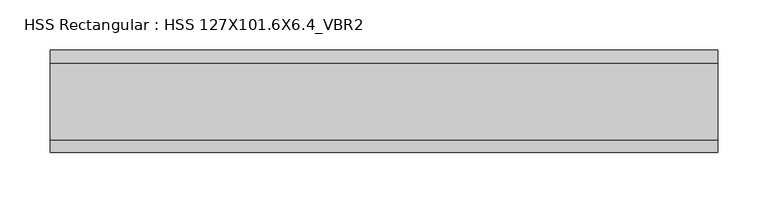
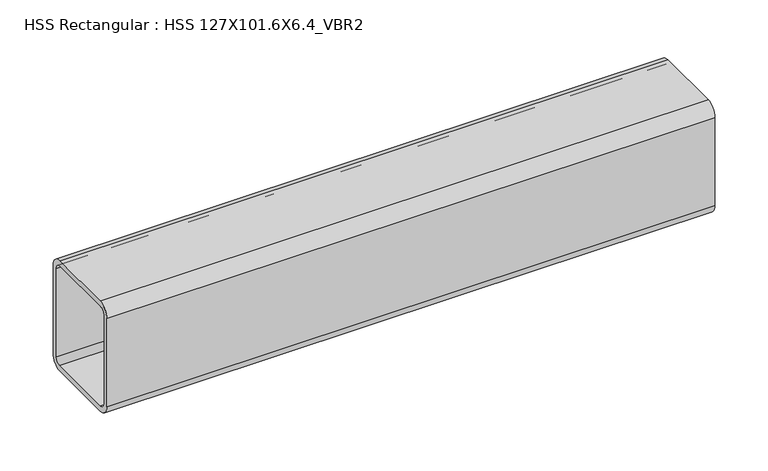
"""IFC4 building model written with IfcOpenShell, lengths in millimetres: member geometry, HSS Rectangular : HSS 127X101.6X6.4_VBR2."""

import ifcopenshell
import ifcopenshell.guid

model = None  # the IFC model being written
_history = None  # IfcOwnerHistory: only IFC2X3 demands one
_inside = {}  # id of a spatial element -> (the spatial element, [elements in it])
_under = {}  # id of a project, library or spatial element -> (it, [spatial elements below it])
_declared = {}  # id of a project -> (the project, [libraries it declares])
_typed = {}  # id of a type object -> (the type object, [elements of that type])
_made_of = {}  # id of a material, layer set ... -> (it, [elements and type objects made of it])


def new_model(schema):
    """Start an empty IFC model of exactly this schema.

    Asked for "IFC4X3", IfcOpenShell would pick the latest addendum, in which some entities
    have other attributes; the version numbers below select the first issue.
    IFC2X3 requires an IfcOwnerHistory on every rooted entity: one is made here for all.
    """
    global model, _history
    if schema == "IFC4X3":
        model = ifcopenshell.file(schema_version=(4, 3, 0, 0))
    else:
        model = ifcopenshell.file(schema=schema)
    _inside.clear()
    _under.clear()
    _declared.clear()
    _typed.clear()
    _made_of.clear()
    _history = None
    if model.schema == "IFC2X3":
        org = make("IfcOrganization", Name="unknown")
        user = make(
            "IfcPersonAndOrganization",
            ThePerson=make("IfcPerson", FamilyName="unknown"),
            TheOrganization=org,
        )
        app = make(
            "IfcApplication",
            ApplicationDeveloper=org,
            Version="unknown",
            ApplicationFullName="unknown",
            ApplicationIdentifier="unknown",
        )
        _history = make(
            "IfcOwnerHistory",
            OwningUser=user,
            OwningApplication=app,
            ChangeAction="ADDED",
            CreationDate=0,
        )
    return model


def make(cls, **values):
    """One entity of the class cls with the attributes given. An attribute that is None is left unset."""
    return model.create_entity(
        cls, **{name: value for name, value in values.items() if value is not None}
    )


def rooted(cls, **values):
    """An entity with a GlobalId (a new one), such as an element, a storey or a relation."""
    return make(cls, GlobalId=ifcopenshell.guid.new(), OwnerHistory=_history, **values)


def si_unit(unit_type, name, prefix=None):
    """IfcSIUnit, for example si_unit("LENGTHUNIT", "METRE", prefix="MILLI")."""
    return make("IfcSIUnit", UnitType=unit_type, Prefix=prefix, Name=name)


def assignment(units):
    """IfcUnitAssignment: the units of a project."""
    return None if units is None else make("IfcUnitAssignment", Units=units)


def point(xyz):
    """IfcCartesianPoint."""
    return None if xyz is None else make("IfcCartesianPoint", Coordinates=xyz)


def direction(xyz):
    """IfcDirection."""
    return None if xyz is None else make("IfcDirection", DirectionRatios=xyz)


def frame(location, z_axis=None, x_axis=None):
    """IfcAxis2Placement3D, a coordinate frame: its origin and axes. An axis left out is left unset."""
    return make(
        "IfcAxis2Placement3D",
        Location=point(location),
        Axis=direction(z_axis),
        RefDirection=direction(x_axis),
    )


def frame_2d(location, x_axis=None):
    """IfcAxis2Placement2D, a coordinate frame in the plane: its origin and x axis."""
    return make(
        "IfcAxis2Placement2D", Location=point(location), RefDirection=direction(x_axis)
    )


def origin():
    """The frame at (0, 0, 0) with its axes left unset."""
    return frame((0.0, 0.0, 0.0))


def place(relative_to, where):
    """IfcLocalPlacement: puts the frame where relative to a parent placement (None: the world)."""
    return make(
        "IfcLocalPlacement", PlacementRelTo=relative_to, RelativePlacement=where
    )


def context(
    kind, dimensions, precision=None, world=None, true_north=None, identifier=None
):
    """IfcGeometricRepresentationContext, for example the 3D "Model" context."""
    return make(
        "IfcGeometricRepresentationContext",
        ContextIdentifier=identifier,
        ContextType=kind,
        CoordinateSpaceDimension=dimensions,
        Precision=precision,
        WorldCoordinateSystem=world,
        TrueNorth=true_north,
    )


def project(units=None, contexts=None):
    """IfcProject with its units and contexts."""
    return rooted(
        "IfcProject",
        Name="project",
        RepresentationContexts=contexts,
        UnitsInContext=assignment(units),
    )


def spatial(cls, under=None, at=None, **own):
    """A site, building, storey or space (cls), placed at a placement, below another one or the project."""
    s = rooted(cls, ObjectPlacement=at, **own)
    if under is not None:
        _under.setdefault(under.id(), (under, []))[1].append(s)
    return s


def polyline(points):
    """IfcPolyline through the points."""
    return make("IfcPolyline", Points=[point(p) for p in points])


def circle_curve(where, radius):
    """IfcCircle in the frame where."""
    return make("IfcCircle", Position=where, Radius=radius)


def trimmed(basis, trim1, trim2, sense, master):
    """IfcTrimmedCurve: the piece of a basis curve between two trims."""
    return make(
        "IfcTrimmedCurve",
        BasisCurve=basis,
        Trim1=trim1,
        Trim2=trim2,
        SenseAgreement=sense,
        MasterRepresentation=master,
    )


def segment(curve, same_sense, transition):
    """IfcCompositeCurveSegment."""
    return make(
        "IfcCompositeCurveSegment",
        Transition=transition,
        SameSense=same_sense,
        ParentCurve=curve,
    )


def composite_curve(segments, self_intersect=None):
    """IfcCompositeCurve: segments joined end to end."""
    return make("IfcCompositeCurve", Segments=segments, SelfIntersect=self_intersect)


def outline(outer, holes=None, kind="AREA"):
    """IfcArbitraryClosedProfileDef: a profile drawn as a closed curve; with holes, ...WithVoids."""
    if holes is None:
        return make("IfcArbitraryClosedProfileDef", ProfileType=kind, OuterCurve=outer)
    return make(
        "IfcArbitraryProfileDefWithVoids",
        ProfileType=kind,
        OuterCurve=outer,
        InnerCurves=holes,
    )


def extrude(swept, where, along, depth):
    """IfcExtrudedAreaSolid: the profile swept, set in the frame where, extruded along a direction by depth."""
    return make(
        "IfcExtrudedAreaSolid",
        SweptArea=swept,
        Position=where,
        ExtrudedDirection=direction(along),
        Depth=depth,
    )


def shape(context_of_items, identifier, shape_type, items):
    """IfcShapeRepresentation: the items that make up one representation, for example the "Body"."""
    return make(
        "IfcShapeRepresentation",
        ContextOfItems=context_of_items,
        RepresentationIdentifier=identifier,
        RepresentationType=shape_type,
        Items=items,
    )


def source(mapping_origin, context_of_items, identifier, shape_type, items):
    """IfcRepresentationMap: a shape defined once, which mapped items show again and again."""
    return make(
        "IfcRepresentationMap",
        MappingOrigin=mapping_origin,
        MappedRepresentation=shape(context_of_items, identifier, shape_type, items),
    )


def transform(
    local_origin,
    x_axis=None,
    y_axis=None,
    z_axis=None,
    scale=None,
    scale2=None,
    scale3=None,
    uniform=True,
):
    """IfcCartesianTransformationOperator3D, or its non-uniform kind. x_axis, y_axis, z_axis: its Axis1, 2, 3."""
    if uniform:
        return make(
            "IfcCartesianTransformationOperator3D",
            Axis1=direction(x_axis),
            Axis2=direction(y_axis),
            LocalOrigin=point(local_origin),
            Scale=scale,
            Axis3=direction(z_axis),
        )
    return make(
        "IfcCartesianTransformationOperator3DnonUniform",
        Axis1=direction(x_axis),
        Axis2=direction(y_axis),
        LocalOrigin=point(local_origin),
        Scale=scale,
        Axis3=direction(z_axis),
        Scale2=scale2,
        Scale3=scale3,
    )


def mapped(mapping_source, mapping_target):
    """IfcMappedItem: shows the shape of a source again, moved by a transform."""
    return make(
        "IfcMappedItem", MappingSource=mapping_source, MappingTarget=mapping_target
    )


def made_of(thing, what):
    """Note that an element or type object is made of a material, layer set ...; save() writes the relation."""
    if what is not None:
        _made_of.setdefault(what.id(), (what, []))[1].append(thing)
    return thing


def element(
    cls,
    number,
    at=None,
    inside=None,
    cuts=None,
    type_object=None,
    material=None,
    context=None,
    identifier="Body",
    shape_type=None,
    held_by="IfcProductDefinitionShape",
    body=None,
    shapes=None,
    **own,
):
    """One element of the class cls, such as IfcWall. Its Tag is "e" and its number.

    at: its placement. inside: the storey or other place that contains it. cuts: it is an
    opening in that element (IfcRelVoidsElement). A single representation is given by context,
    identifier, shape_type and body (its items); several are given by shapes. held_by: the class
    of the entity that holds the representations. save() writes the other relations.
    """
    e = rooted(cls, Tag="e%d" % number, ObjectPlacement=at, **own)
    if body is not None:
        shapes = [shape(context, identifier, shape_type, body)]
    if shapes is not None:
        e.Representation = make(held_by, Representations=shapes)
    if inside is not None:
        _inside.setdefault(inside.id(), (inside, []))[1].append(e)
    if cuts is not None:
        rooted(
            "IfcRelVoidsElement", RelatingBuildingElement=cuts, RelatedOpeningElement=e
        )
    if type_object is not None:
        _typed.setdefault(type_object.id(), (type_object, []))[1].append(e)
    return made_of(e, material)


def aggregate(whole, parts):
    """IfcRelAggregates: a whole, such as a stair, and the parts it consists of."""
    return rooted("IfcRelAggregates", RelatingObject=whole, RelatedObjects=parts)


def save(model, path):
    """Write the relations noted so far, then the file.

    IfcRelAggregates (storeys below a building ...), IfcRelContainedInSpatialStructure (elements
    in a storey), IfcRelDefinesByType, IfcRelAssociatesMaterial and IfcRelDeclares: one each for
    every whole, place, type object, material and project.
    """
    for whole, parts in _under.values():
        aggregate(whole, parts)
    for where, things in _inside.values():
        rooted(
            "IfcRelContainedInSpatialStructure",
            RelatedElements=things,
            RelatingStructure=where,
        )
    for kind, things in _typed.values():
        rooted("IfcRelDefinesByType", RelatedObjects=things, RelatingType=kind)
    for what, things in _made_of.values():
        rooted("IfcRelAssociatesMaterial", RelatedObjects=things, RelatingMaterial=what)
    for by, libraries in _declared.values():
        rooted("IfcRelDeclares", RelatingContext=by, RelatedDefinitions=libraries)
    model.write(path)


def hss_rectangular_hss_127x101_6x6_4_vbr2_0ae2a549(model_context):
    return source(origin(), model_context, "Body", "SweptSolid", [
        extrude(outline(composite_curve([segment(polyline([(50.8, 50.8), (50.8, -50.8)]), True, "CONTINUOUS"), segment(trimmed(circle_curve(frame_2d((38.1, -50.8)), 12.7), [point((50.8, -50.8))], [point((38.1, -63.5))], False, "CARTESIAN"), True, "CONTINUOUS"), segment(polyline([(38.1, -63.5), (-38.1, -63.5)]), True, "CONTINUOUS"), segment(trimmed(circle_curve(frame_2d((-38.1, -50.8)), 12.7), [point((-38.1, -63.5))], [point((-50.8, -50.8))], False, "CARTESIAN"), True, "CONTINUOUS"), segment(polyline([(-50.8, -50.8), (-50.8, 50.8)]), True, "CONTINUOUS"), segment(trimmed(circle_curve(frame_2d((-38.1, 50.8)), 12.7), [point((-50.8, 50.8))], [point((-38.1, 63.5))], False, "CARTESIAN"), True, "CONTINUOUS"), segment(polyline([(-38.1, 63.5), (38.1, 63.5)]), True, "CONTINUOUS"), segment(trimmed(circle_curve(frame_2d((38.1, 50.8)), 12.7), [point((38.1, 63.5))], [point((50.8, 50.8))], False, "CARTESIAN"), True, "CONTINUOUS")], self_intersect=False), holes=[composite_curve([segment(trimmed(circle_curve(frame_2d((-38.1, 50.8)), 6.35), [point((-38.1, 57.15))], [point((-44.45, 50.8))], True, "CARTESIAN"), True, "CONTINUOUS"), segment(polyline([(-44.45, 50.8), (-44.45, -50.8)]), True, "CONTINUOUS"), segment(trimmed(circle_curve(frame_2d((-38.1, -50.8)), 6.35), [point((-44.45, -50.8))], [point((-38.1, -57.15))], True, "CARTESIAN"), True, "CONTINUOUS"), segment(polyline([(-38.1, -57.15), (38.1, -57.15)]), True, "CONTINUOUS"), segment(trimmed(circle_curve(frame_2d((38.1, -50.8)), 6.35), [point((38.1, -57.15))], [point((44.45, -50.8))], True, "CARTESIAN"), True, "CONTINUOUS"), segment(polyline([(44.45, -50.8), (44.45, 50.8)]), True, "CONTINUOUS"), segment(trimmed(circle_curve(frame_2d((38.1, 50.8)), 6.35), [point((44.45, 50.8))], [point((38.1, 57.15))], True, "CARTESIAN"), True, "CONTINUOUS"), segment(polyline([(38.1, 57.15), (-38.1, 57.15)]), True, "CONTINUOUS")], self_intersect=False)]), frame((-347.6762066, 0.0, 0.0), z_axis=(1.0, 0.0, 0.0), x_axis=(0.0, 1.0, 0.0)), (0.0, 0.0, 1.0), 661.6356249),
    ])


if __name__ == "__main__":
    model = new_model("IFC4")
    model_context = context("Model", 3, world=origin())
    ifc_project = project(units=[si_unit("LENGTHUNIT", "METRE", prefix="MILLI")], contexts=[model_context])
    site = spatial("IfcSite", under=ifc_project)
    building = spatial("IfcBuilding", under=site)
    placement = place(None, origin())
    hss_rectangular_hss_127x101_6x6_4_vbr2_shape = hss_rectangular_hss_127x101_6x6_4_vbr2_0ae2a549(model_context)
    element("IfcMember", 1, ObjectType="HSS Rectangular : HSS 127X101.6X6.4_VBR2", at=placement, inside=building, context=model_context, shape_type="MappedRepresentation", body=[
        mapped(hss_rectangular_hss_127x101_6x6_4_vbr2_shape, transform((0.0, 0.0, 0.0), x_axis=(1.0, 0.0, 0.0), y_axis=(0.0, 1.0, 0.0), z_axis=(0.0, 0.0, 1.0))),
    ])
    save(model, "model.ifc")

# Revit data of these elements
# Type "HSS Rectangular : HSS 127X101.6X6.4_VBR2"
#   Section Name Key = "HSS5X4X1/4"
#   Assembly Code = "B10"
#   Width = 10.16 cm
#   Wall Nominal Thickness = 0.635 cm
#   Wall Design Thickness = 0.5918 cm
#   Torsional Moment of Inertia = 749.217 cm⁴
#   Torsional Modulus = 136.34 cm³
#   Section Area = 24.7741 cm²
#   Plastic Modulus weak axis = 91.2759 cm³
#   Plastic Modulus strong axis = 106.352 cm³
#   Perimeter = 0.435254 m²/m
#   Outer Fillet = 1.27 cm
#   Nominal Weight = 20.7004 kgf/m
#   Moment of Inertia weak axis = 393.755 cm⁴
#   Moment of Inertia strong axis = 557.75 cm⁴
#   Inner Fillet = 0.635 cm
#   Height = 12.7 cm
#   Elastic Modulus weak axis = 77.5108 cm³
#   Elastic Modulus strong axis = 87.6708 cm³
#   Centroid Vertical = 6.35 cm
#   Centroid Horizontal = 5.08 cm
#   Length [instance default] = 1524 mm
#   Structural Material [instance default] = Steel ASTM A500, Grade C, Rectangular and Square
#   Principal Axes Angle = 0
# Element 1 (IfcMember, "HSS Rectangular : HSS 127X101.6X6.4_VBR2")
#   Materials on its faces: "Steel ASTM A500, Grade C, Rectangular and Square"
# Materials
#   "Steel ASTM A500, Grade C, Rectangular and Square": class "Metal", colour RGB 120 120 120, transparency 0, Description = "Carbon steel", Cost = 0
